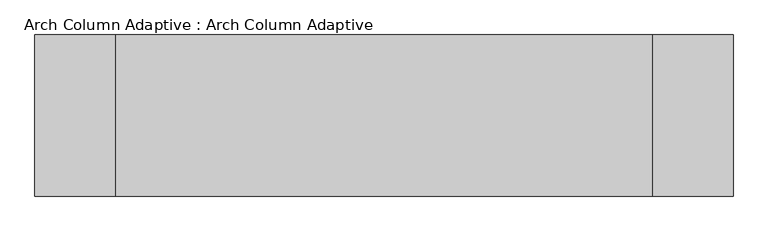
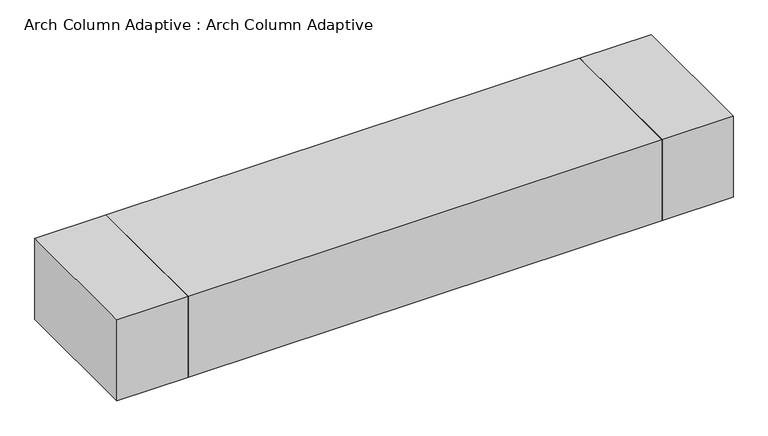
"""IFC4 building model written with IfcOpenShell, lengths in millimetres: proxy geometry, Arch Column Adaptive : Arch Column Adaptive."""

from ifc_helpers import new_model, si_unit, frame, origin, place, context, project, spatial, polyline, outline, extrude, source, transform, mapped, element, save


def arch_column_adaptive_arch_column_adaptive_99ff4f7a(model_context):
    return source(origin(), model_context, "Body", "SweptSolid", [
        extrude(outline(polyline([(5000.0, -1500.0), (5000.0, 1500.0), (6500.0, 1500.0), (6500.0, -1500.0), (5000.0, -1500.0)])), frame((0.0, 0.0, 22790.0), z_axis=(0.0, 0.0, 1.0), x_axis=(1.0, 0.0, 0.0)), (0.0, 0.0, 1.0), 1800.0),
        extrude(outline(polyline([(-5000.0, 1500.0), (-5000.0, -1500.0), (-6500.0, -1500.0), (-6500.0, 1500.0), (-5000.0, 1500.0)])), frame((0.0, 0.0, 22790.0), z_axis=(0.0, 0.0, 1.0), x_axis=(1.0, 0.0, 0.0)), (0.0, 0.0, 1.0), 1800.0),
        extrude(outline(polyline([(-5000.0, -1500.0), (-5000.0, 1500.0), (5000.0, 1500.0), (5000.0, -1500.0), (-5000.0, -1500.0)])), frame((0.0, 0.0, 22790.0), z_axis=(0.0, 0.0, 1.0), x_axis=(1.0, 0.0, 0.0)), (0.0, 0.0, 1.0), 1800.0),
    ])


if __name__ == "__main__":
    model = new_model("IFC4")
    model_context = context("Model", 3, world=origin())
    ifc_project = project(units=[si_unit("LENGTHUNIT", "METRE", prefix="MILLI")], contexts=[model_context])
    site = spatial("IfcSite", under=ifc_project)
    building = spatial("IfcBuilding", under=site)
    placement = place(None, origin())
    arch_column_adaptive_arch_column_adaptive_shape = arch_column_adaptive_arch_column_adaptive_99ff4f7a(model_context)
    element("IfcBuildingElementProxy", 1, Name="Arch Column Adaptive : Arch Column Adaptive", ObjectType="Arch Column Adaptive : Arch Column Adaptive", at=placement, inside=building, context=model_context, shape_type="MappedRepresentation", body=[
        mapped(arch_column_adaptive_arch_column_adaptive_shape, transform((0.0, 0.0, 0.0), x_axis=(1.0, 0.0, 0.0), y_axis=(0.0, 1.0, 0.0), z_axis=(0.0, 0.0, 1.0))),
    ])
    save(model, "model.ifc")

# Revit data of these elements
# Type "Arch Column Adaptive : Arch Column Adaptive"
#   Top Width = 3000 mm
#   Length [instance default] = 21000 mm
#   Height [instance default] = 50000 mm
#   Default Elevation = 0
# Element 1 (IfcBuildingElementProxy, "Arch Column Adaptive : Arch Column Adaptive")
#   Height = 22790 mm
